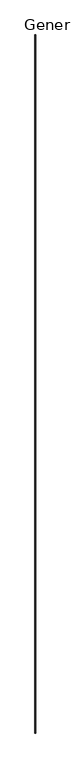
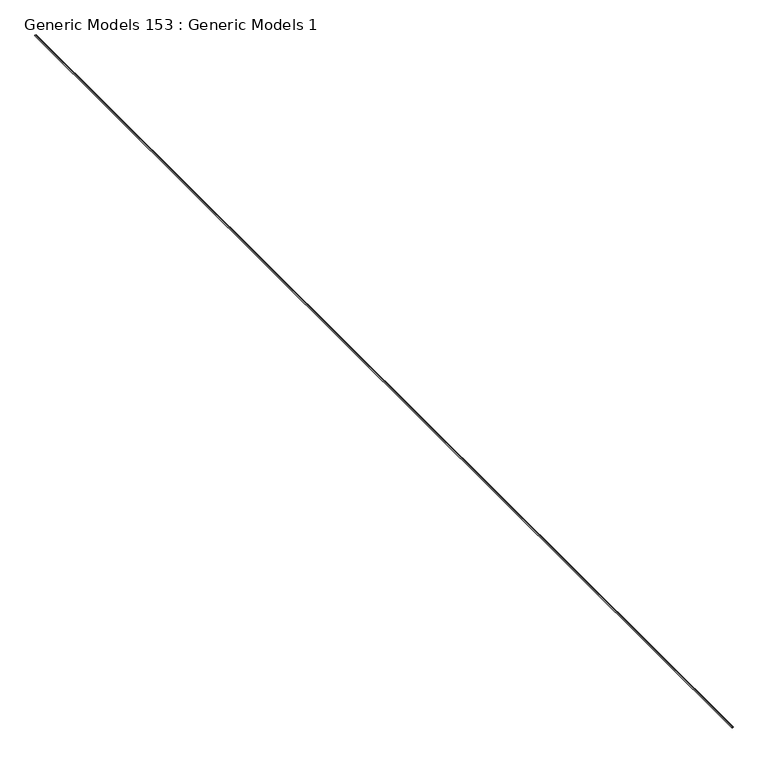
"""IFC4 building model written with IfcOpenShell, lengths in millimetres: proxy geometry, Generic Models 153 : Generic Models 1."""

import ifcopenshell
import ifcopenshell.guid

model = None  # the IFC model being written
_history = None  # IfcOwnerHistory: only IFC2X3 demands one
_inside = {}  # id of a spatial element -> (the spatial element, [elements in it])
_under = {}  # id of a project, library or spatial element -> (it, [spatial elements below it])
_declared = {}  # id of a project -> (the project, [libraries it declares])
_typed = {}  # id of a type object -> (the type object, [elements of that type])
_made_of = {}  # id of a material, layer set ... -> (it, [elements and type objects made of it])


def new_model(schema):
    """Start an empty IFC model of exactly this schema.

    Asked for "IFC4X3", IfcOpenShell would pick the latest addendum, in which some entities
    have other attributes; the version numbers below select the first issue.
    IFC2X3 requires an IfcOwnerHistory on every rooted entity: one is made here for all.
    """
    global model, _history
    if schema == "IFC4X3":
        model = ifcopenshell.file(schema_version=(4, 3, 0, 0))
    else:
        model = ifcopenshell.file(schema=schema)
    _inside.clear()
    _under.clear()
    _declared.clear()
    _typed.clear()
    _made_of.clear()
    _history = None
    if model.schema == "IFC2X3":
        org = make("IfcOrganization", Name="unknown")
        user = make(
            "IfcPersonAndOrganization",
            ThePerson=make("IfcPerson", FamilyName="unknown"),
            TheOrganization=org,
        )
        app = make(
            "IfcApplication",
            ApplicationDeveloper=org,
            Version="unknown",
            ApplicationFullName="unknown",
            ApplicationIdentifier="unknown",
        )
        _history = make(
            "IfcOwnerHistory",
            OwningUser=user,
            OwningApplication=app,
            ChangeAction="ADDED",
            CreationDate=0,
        )
    return model


def make(cls, **values):
    """One entity of the class cls with the attributes given. An attribute that is None is left unset."""
    return model.create_entity(
        cls, **{name: value for name, value in values.items() if value is not None}
    )


def rooted(cls, **values):
    """An entity with a GlobalId (a new one), such as an element, a storey or a relation."""
    return make(cls, GlobalId=ifcopenshell.guid.new(), OwnerHistory=_history, **values)


def si_unit(unit_type, name, prefix=None):
    """IfcSIUnit, for example si_unit("LENGTHUNIT", "METRE", prefix="MILLI")."""
    return make("IfcSIUnit", UnitType=unit_type, Prefix=prefix, Name=name)


def assignment(units):
    """IfcUnitAssignment: the units of a project."""
    return None if units is None else make("IfcUnitAssignment", Units=units)


def point(xyz):
    """IfcCartesianPoint."""
    return None if xyz is None else make("IfcCartesianPoint", Coordinates=xyz)


def direction(xyz):
    """IfcDirection."""
    return None if xyz is None else make("IfcDirection", DirectionRatios=xyz)


def frame(location, z_axis=None, x_axis=None):
    """IfcAxis2Placement3D, a coordinate frame: its origin and axes. An axis left out is left unset."""
    return make(
        "IfcAxis2Placement3D",
        Location=point(location),
        Axis=direction(z_axis),
        RefDirection=direction(x_axis),
    )


def origin():
    """The frame at (0, 0, 0) with its axes left unset."""
    return frame((0.0, 0.0, 0.0))


def place(relative_to, where):
    """IfcLocalPlacement: puts the frame where relative to a parent placement (None: the world)."""
    return make(
        "IfcLocalPlacement", PlacementRelTo=relative_to, RelativePlacement=where
    )


def context(
    kind, dimensions, precision=None, world=None, true_north=None, identifier=None
):
    """IfcGeometricRepresentationContext, for example the 3D "Model" context."""
    return make(
        "IfcGeometricRepresentationContext",
        ContextIdentifier=identifier,
        ContextType=kind,
        CoordinateSpaceDimension=dimensions,
        Precision=precision,
        WorldCoordinateSystem=world,
        TrueNorth=true_north,
    )


def project(units=None, contexts=None):
    """IfcProject with its units and contexts."""
    return rooted(
        "IfcProject",
        Name="project",
        RepresentationContexts=contexts,
        UnitsInContext=assignment(units),
    )


def spatial(cls, under=None, at=None, **own):
    """A site, building, storey or space (cls), placed at a placement, below another one or the project."""
    s = rooted(cls, ObjectPlacement=at, **own)
    if under is not None:
        _under.setdefault(under.id(), (under, []))[1].append(s)
    return s


def polyline(points):
    """IfcPolyline through the points."""
    return make("IfcPolyline", Points=[point(p) for p in points])


def circle_curve(where, radius):
    """IfcCircle in the frame where."""
    return make("IfcCircle", Position=where, Radius=radius)


def ellipse_curve(where, semi_axis1, semi_axis2):
    """IfcEllipse in the frame where."""
    return make(
        "IfcEllipse", Position=where, SemiAxis1=semi_axis1, SemiAxis2=semi_axis2
    )


def trimmed(basis, trim1, trim2, sense, master):
    """IfcTrimmedCurve: the piece of a basis curve between two trims."""
    return make(
        "IfcTrimmedCurve",
        BasisCurve=basis,
        Trim1=trim1,
        Trim2=trim2,
        SenseAgreement=sense,
        MasterRepresentation=master,
    )


def shape(context_of_items, identifier, shape_type, items):
    """IfcShapeRepresentation: the items that make up one representation, for example the "Body"."""
    return make(
        "IfcShapeRepresentation",
        ContextOfItems=context_of_items,
        RepresentationIdentifier=identifier,
        RepresentationType=shape_type,
        Items=items,
    )


def source(mapping_origin, context_of_items, identifier, shape_type, items):
    """IfcRepresentationMap: a shape defined once, which mapped items show again and again."""
    return make(
        "IfcRepresentationMap",
        MappingOrigin=mapping_origin,
        MappedRepresentation=shape(context_of_items, identifier, shape_type, items),
    )


def transform(
    local_origin,
    x_axis=None,
    y_axis=None,
    z_axis=None,
    scale=None,
    scale2=None,
    scale3=None,
    uniform=True,
):
    """IfcCartesianTransformationOperator3D, or its non-uniform kind. x_axis, y_axis, z_axis: its Axis1, 2, 3."""
    if uniform:
        return make(
            "IfcCartesianTransformationOperator3D",
            Axis1=direction(x_axis),
            Axis2=direction(y_axis),
            LocalOrigin=point(local_origin),
            Scale=scale,
            Axis3=direction(z_axis),
        )
    return make(
        "IfcCartesianTransformationOperator3DnonUniform",
        Axis1=direction(x_axis),
        Axis2=direction(y_axis),
        LocalOrigin=point(local_origin),
        Scale=scale,
        Axis3=direction(z_axis),
        Scale2=scale2,
        Scale3=scale3,
    )


def mapped(mapping_source, mapping_target):
    """IfcMappedItem: shows the shape of a source again, moved by a transform."""
    return make(
        "IfcMappedItem", MappingSource=mapping_source, MappingTarget=mapping_target
    )


def made_of(thing, what):
    """Note that an element or type object is made of a material, layer set ...; save() writes the relation."""
    if what is not None:
        _made_of.setdefault(what.id(), (what, []))[1].append(thing)
    return thing


def element(
    cls,
    number,
    at=None,
    inside=None,
    cuts=None,
    type_object=None,
    material=None,
    context=None,
    identifier="Body",
    shape_type=None,
    held_by="IfcProductDefinitionShape",
    body=None,
    shapes=None,
    **own,
):
    """One element of the class cls, such as IfcWall. Its Tag is "e" and its number.

    at: its placement. inside: the storey or other place that contains it. cuts: it is an
    opening in that element (IfcRelVoidsElement). A single representation is given by context,
    identifier, shape_type and body (its items); several are given by shapes. held_by: the class
    of the entity that holds the representations. save() writes the other relations.
    """
    e = rooted(cls, Tag="e%d" % number, ObjectPlacement=at, **own)
    if body is not None:
        shapes = [shape(context, identifier, shape_type, body)]
    if shapes is not None:
        e.Representation = make(held_by, Representations=shapes)
    if inside is not None:
        _inside.setdefault(inside.id(), (inside, []))[1].append(e)
    if cuts is not None:
        rooted(
            "IfcRelVoidsElement", RelatingBuildingElement=cuts, RelatedOpeningElement=e
        )
    if type_object is not None:
        _typed.setdefault(type_object.id(), (type_object, []))[1].append(e)
    return made_of(e, material)


def aggregate(whole, parts):
    """IfcRelAggregates: a whole, such as a stair, and the parts it consists of."""
    return rooted("IfcRelAggregates", RelatingObject=whole, RelatedObjects=parts)


def save(model, path):
    """Write the relations noted so far, then the file.

    IfcRelAggregates (storeys below a building ...), IfcRelContainedInSpatialStructure (elements
    in a storey), IfcRelDefinesByType, IfcRelAssociatesMaterial and IfcRelDeclares: one each for
    every whole, place, type object, material and project.
    """
    for whole, parts in _under.values():
        aggregate(whole, parts)
    for where, things in _inside.values():
        rooted(
            "IfcRelContainedInSpatialStructure",
            RelatedElements=things,
            RelatingStructure=where,
        )
    for kind, things in _typed.values():
        rooted("IfcRelDefinesByType", RelatedObjects=things, RelatingType=kind)
    for what, things in _made_of.values():
        rooted("IfcRelAssociatesMaterial", RelatedObjects=things, RelatingMaterial=what)
    for by, libraries in _declared.values():
        rooted("IfcRelDeclares", RelatingContext=by, RelatedDefinitions=libraries)
    model.write(path)


def plane_surface(at):
    """IfcPlane: the flat surface through the origin of the frame at, square to its z axis."""
    return make("IfcPlane", Position=at)


def cylinder_surface(at, radius):
    """IfcCylindricalSurface: all points at the distance radius from the z axis of the frame at."""
    return make("IfcCylindricalSurface", Position=at, Radius=radius)


def revolved_surface(curve, axis_point, axis_direction):
    """IfcSurfaceOfRevolution: the curve turned about the line through axis_point along axis_direction."""
    return make(
        "IfcSurfaceOfRevolution",
        SweptCurve=make("IfcArbitraryOpenProfileDef", ProfileType="CURVE", Curve=curve),
        AxisPosition=make("IfcAxis1Placement", Location=point(axis_point), Axis=direction(axis_direction)),
    )


def extruded_surface(curve, direction_of_extrusion, depth):
    """IfcSurfaceOfLinearExtrusion: the curve pushed along a direction by depth."""
    return make(
        "IfcSurfaceOfLinearExtrusion",
        SweptCurve=make("IfcArbitraryOpenProfileDef", ProfileType="CURVE", Curve=curve),
        ExtrudedDirection=direction(direction_of_extrusion),
        Depth=depth,
    )


def advanced_brep(points, edges, surfaces, faces):
    """IfcAdvancedBrep: a solid bounded by faces that lie on surfaces and meet in shared edges.

    An edge is (start, end): straight between two places in points (the first is 0);
    or (start, end, curve); or (start, end, curve, False) where it runs against its curve.
    A face is (place in surfaces, loops), or (place, loops, False) where it looks against
    its surface's normal. A loop lists edges by number (the first is 1), with a minus sign
    where the edge is run from its end to its start. The first loop is the outer one.
    """
    corners = [point(p) for p in points]
    vertices = [make("IfcVertexPoint", VertexGeometry=c) for c in corners]
    made = []
    for start, end, *more in edges:
        made.append(
            make(
                "IfcEdgeCurve",
                EdgeStart=vertices[start],
                EdgeEnd=vertices[end],
                EdgeGeometry=more[0] if more else make("IfcPolyline", Points=[corners[start], corners[end]]),
                SameSense=more[1] if len(more) > 1 else True,
            )
        )
    hull = []
    for where, loops, *sense in faces:
        bounds = []
        for j, loop in enumerate(loops):
            ring = [make("IfcOrientedEdge", EdgeElement=made[abs(k) - 1], Orientation=k > 0) for k in loop]
            bounds.append(
                make(
                    "IfcFaceOuterBound" if j == 0 else "IfcFaceBound",
                    Bound=make("IfcEdgeLoop", EdgeList=ring),
                    Orientation=True,
                )
            )
        hull.append(make("IfcAdvancedFace", Bounds=bounds, FaceSurface=surfaces[where], SameSense=sense[0] if sense else True))
    return make("IfcAdvancedBrep", Outer=make("IfcClosedShell", CfsFaces=hull))


def generic_models_153_generic_models_1_efdc0eff(model_context):
    return source(origin(), model_context, "Body", "AdvancedBrep", [
        advanced_brep(
        [(-6512.6410252, 11981.8769662, 126183.5628287), (-6517.4035252, 11981.8769662, 126183.5628287), (-6518.8311642, 11981.8769662, 126185.4688165), (-6518.8311642, 11981.8769662, 126191.1818409), (-6517.4035252, 11981.8769662, 126193.0878287), (-6512.6410252, 11981.8769662, 126193.0878287), (-6512.6410252, -7068.1230338, 126183.5628287), (-6512.6410252, -7068.1230338, 126193.0878287), (-6517.4035252, -7068.1230338, 126193.0878287), (-6518.8311642, -7068.1230338, 126191.1818409), (-6518.8311642, -7068.1230338, 126185.4688165), (-6517.4035252, -7068.1230338, 126183.5628287)],
        [
            (0, 1),
            (1, 2, circle_curve(frame((-6513.0314145, 11981.8769662, 126188.3253287), z_axis=(0.0, 1.0, 0.0), x_axis=(0.0, 0.0, -1.0)), 6.4650413)),
            (2, 3, ellipse_curve(frame((-6524.5472752, 11981.8769662, 126188.3253287), z_axis=(0.0, 1.0, 0.0), x_axis=(1.0, 0.0, 0.0)), 7.14375, 4.7625)),
            (3, 4, circle_curve(frame((-6513.0314145, 11981.8769662, 126188.3253287), z_axis=(0.0, 1.0, 0.0), x_axis=(0.0, 0.0, -1.0)), 6.4650413)),
            (4, 5),
            (5, 0, circle_curve(frame((-6508.2689145, 11981.8769662, 126188.3253287), z_axis=(0.0, -1.0, 0.0), x_axis=(0.0, 0.0, -1.0)), 6.4650413)),
            (6, 7, circle_curve(frame((-6508.2689145, -7068.1230338, 126188.3253287), z_axis=(0.0, 1.0, 0.0), x_axis=(0.0, 0.0, -1.0)), 6.4650413)),
            (7, 8),
            (8, 9, circle_curve(frame((-6513.0314145, -7068.1230338, 126188.3253287), z_axis=(0.0, -1.0, 0.0), x_axis=(0.0, 0.0, -1.0)), 6.4650413)),
            (9, 10, ellipse_curve(frame((-6524.5472752, -7068.1230338, 126188.3253287), z_axis=(0.0, -1.0, 0.0), x_axis=(1.0, 0.0, 0.0)), 7.14375, 4.7625)),
            (10, 11, circle_curve(frame((-6513.0314145, -7068.1230338, 126188.3253287), z_axis=(0.0, -1.0, 0.0), x_axis=(0.0, 0.0, -1.0)), 6.4650413)),
            (11, 6),
            (2, 10),
            (9, 3),
            (5, 7),
            (6, 0),
            (4, 8),
            (1, 11),
        ],
        [
            plane_surface(frame((-6512.6410252, 11981.8769662, 126193.0878287), z_axis=(0.0, 1.0, 0.0), x_axis=(1.0, 0.0, 0.0))),
            plane_surface(frame((-6512.6410252, -7068.1230338, 126193.0878287), z_axis=(0.0, -1.0, 0.0), x_axis=(1.0, 0.0, 0.0))),
            extruded_surface(trimmed(ellipse_curve(frame((-6524.5472752, -7068.1230338, 126188.3253287), z_axis=(0.0, 1.0, 0.0), x_axis=(1.0, 0.0, 0.0)), 7.14375, 4.7625), [point((-6518.8311642, -7068.1230338, 126185.4688165))], [point((-6518.8311642, -7068.1230338, 126191.1818409))], True, "CARTESIAN"), (0.0, 19050.0, 0.0), 19050.0),
            revolved_surface(polyline([(-6508.2689145, -7068.1230338000005, 126181.86028739999), (-6508.2689145, 11981.8769662, 126181.86028739999)]), (-6508.2689145, 11981.8769662, 126188.3253287), (0.0, -1.0, 0.0)),
            plane_surface(frame((-6517.4035252, 11981.8769662, 126193.0878287), z_axis=(0.0, 0.0, 1.0), x_axis=(0.0, -1.0, 0.0))),
            cylinder_surface(frame((-6513.0314145, 11981.8769662, 126188.3253287), z_axis=(0.0, 1.0, 0.0), x_axis=(0.0, 0.0, -1.0)), 6.4650413),
            plane_surface(frame((-6512.6410252, 11981.8769662, 126183.5628287), z_axis=(0.0, 0.0, -1.0), x_axis=(0.0, -1.0, 0.0))),
        ],
        [
            (0, [[1, 2, 3, 4, 5, 6]]),
            (1, [[7, 8, 9, 10, 11, 12]]),
            (2, [[-3, 13, -10, 14]]),
            (3, [[-6, 15, -7, 16]]),
            (4, [[-5, 17, -8, -15]]),
            (5, [[-4, -14, -9, -17]]),
            (5, [[-2, 18, -11, -13]]),
            (6, [[-1, -16, -12, -18]]),
        ],
    ),
    ])


if __name__ == "__main__":
    model = new_model("IFC4")
    model_context = context("Model", 3, world=origin())
    ifc_project = project(units=[si_unit("LENGTHUNIT", "METRE", prefix="MILLI")], contexts=[model_context])
    site = spatial("IfcSite", under=ifc_project)
    building = spatial("IfcBuilding", under=site)
    placement = place(None, origin())
    generic_models_153_generic_models_1_shape = generic_models_153_generic_models_1_efdc0eff(model_context)
    element("IfcBuildingElementProxy", 1, Name="Generic Models 153 : Generic Models 1", ObjectType="Generic Models 153 : Generic Models 1", at=placement, inside=building, context=model_context, shape_type="MappedRepresentation", body=[
        mapped(generic_models_153_generic_models_1_shape, transform((0.0, 0.0, 0.0), x_axis=(1.0, 0.0, 0.0), y_axis=(0.0, 1.0, 0.0), z_axis=(0.0, 0.0, 1.0))),
    ])
    save(model, "model.ifc")

# Revit data of these elements
# Element 1 (IfcBuildingElementProxy, "Generic Models 153 : Generic Models 1")
#   Materials on its faces: "_SEALANT AND BACKROD, IF NECESSARY"
# Materials
#   "_SEALANT AND BACKROD, IF NECESSARY": class "Generic", colour RGB 190 220 196, transparency 0, Cost = 0
